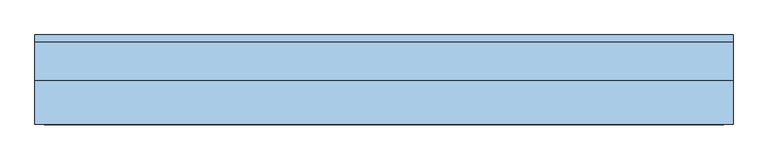
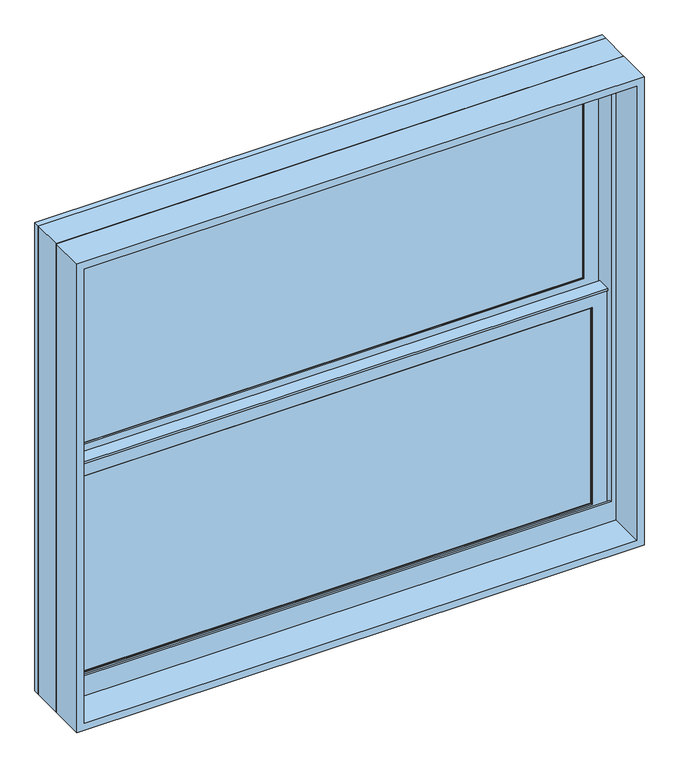
"""IFC4 building model written with IfcOpenShell, lengths in millimetres: window geometry, Window-Double_Hung-Marvin-Essential : ESDH4036."""

import ifcopenshell
import ifcopenshell.guid

model = None  # the IFC model being written
_history = None  # IfcOwnerHistory: only IFC2X3 demands one
_inside = {}  # id of a spatial element -> (the spatial element, [elements in it])
_under = {}  # id of a project, library or spatial element -> (it, [spatial elements below it])
_declared = {}  # id of a project -> (the project, [libraries it declares])
_typed = {}  # id of a type object -> (the type object, [elements of that type])
_made_of = {}  # id of a material, layer set ... -> (it, [elements and type objects made of it])


def new_model(schema):
    """Start an empty IFC model of exactly this schema.

    Asked for "IFC4X3", IfcOpenShell would pick the latest addendum, in which some entities
    have other attributes; the version numbers below select the first issue.
    IFC2X3 requires an IfcOwnerHistory on every rooted entity: one is made here for all.
    """
    global model, _history
    if schema == "IFC4X3":
        model = ifcopenshell.file(schema_version=(4, 3, 0, 0))
    else:
        model = ifcopenshell.file(schema=schema)
    _inside.clear()
    _under.clear()
    _declared.clear()
    _typed.clear()
    _made_of.clear()
    _history = None
    if model.schema == "IFC2X3":
        org = make("IfcOrganization", Name="unknown")
        user = make(
            "IfcPersonAndOrganization",
            ThePerson=make("IfcPerson", FamilyName="unknown"),
            TheOrganization=org,
        )
        app = make(
            "IfcApplication",
            ApplicationDeveloper=org,
            Version="unknown",
            ApplicationFullName="unknown",
            ApplicationIdentifier="unknown",
        )
        _history = make(
            "IfcOwnerHistory",
            OwningUser=user,
            OwningApplication=app,
            ChangeAction="ADDED",
            CreationDate=0,
        )
    return model


def make(cls, **values):
    """One entity of the class cls with the attributes given. An attribute that is None is left unset."""
    return model.create_entity(
        cls, **{name: value for name, value in values.items() if value is not None}
    )


def rooted(cls, **values):
    """An entity with a GlobalId (a new one), such as an element, a storey or a relation."""
    return make(cls, GlobalId=ifcopenshell.guid.new(), OwnerHistory=_history, **values)


def si_unit(unit_type, name, prefix=None):
    """IfcSIUnit, for example si_unit("LENGTHUNIT", "METRE", prefix="MILLI")."""
    return make("IfcSIUnit", UnitType=unit_type, Prefix=prefix, Name=name)


def assignment(units):
    """IfcUnitAssignment: the units of a project."""
    return None if units is None else make("IfcUnitAssignment", Units=units)


def point(xyz):
    """IfcCartesianPoint."""
    return None if xyz is None else make("IfcCartesianPoint", Coordinates=xyz)


def direction(xyz):
    """IfcDirection."""
    return None if xyz is None else make("IfcDirection", DirectionRatios=xyz)


def frame(location, z_axis=None, x_axis=None):
    """IfcAxis2Placement3D, a coordinate frame: its origin and axes. An axis left out is left unset."""
    return make(
        "IfcAxis2Placement3D",
        Location=point(location),
        Axis=direction(z_axis),
        RefDirection=direction(x_axis),
    )


def origin():
    """The frame at (0, 0, 0) with its axes left unset."""
    return frame((0.0, 0.0, 0.0))


def place(relative_to, where):
    """IfcLocalPlacement: puts the frame where relative to a parent placement (None: the world)."""
    return make(
        "IfcLocalPlacement", PlacementRelTo=relative_to, RelativePlacement=where
    )


def context(
    kind, dimensions, precision=None, world=None, true_north=None, identifier=None
):
    """IfcGeometricRepresentationContext, for example the 3D "Model" context."""
    return make(
        "IfcGeometricRepresentationContext",
        ContextIdentifier=identifier,
        ContextType=kind,
        CoordinateSpaceDimension=dimensions,
        Precision=precision,
        WorldCoordinateSystem=world,
        TrueNorth=true_north,
    )


def project(units=None, contexts=None):
    """IfcProject with its units and contexts."""
    return rooted(
        "IfcProject",
        Name="project",
        RepresentationContexts=contexts,
        UnitsInContext=assignment(units),
    )


def spatial(cls, under=None, at=None, **own):
    """A site, building, storey or space (cls), placed at a placement, below another one or the project."""
    s = rooted(cls, ObjectPlacement=at, **own)
    if under is not None:
        _under.setdefault(under.id(), (under, []))[1].append(s)
    return s


def polyline(points):
    """IfcPolyline through the points."""
    return make("IfcPolyline", Points=[point(p) for p in points])


def outline(outer, holes=None, kind="AREA"):
    """IfcArbitraryClosedProfileDef: a profile drawn as a closed curve; with holes, ...WithVoids."""
    if holes is None:
        return make("IfcArbitraryClosedProfileDef", ProfileType=kind, OuterCurve=outer)
    return make(
        "IfcArbitraryProfileDefWithVoids",
        ProfileType=kind,
        OuterCurve=outer,
        InnerCurves=holes,
    )


def extrude(swept, where, along, depth):
    """IfcExtrudedAreaSolid: the profile swept, set in the frame where, extruded along a direction by depth."""
    return make(
        "IfcExtrudedAreaSolid",
        SweptArea=swept,
        Position=where,
        ExtrudedDirection=direction(along),
        Depth=depth,
    )


def faces_of(points, faces, orient=None, outer=None):
    """IfcFace entities. A face is a list of loops; a loop is a list of indices into points, from 0.

    orient and outer hold one flag for each loop. By default every Orientation is true, the
    first loop of a face is its IfcFaceOuterBound and the others are IfcFaceBound.
    """
    made = []
    for i, loops in enumerate(faces):
        bounds = []
        for j, loop in enumerate(loops):
            is_outer = j == 0 if outer is None else outer[i][j]
            bounds.append(
                make(
                    "IfcFaceOuterBound" if is_outer else "IfcFaceBound",
                    Bound=make("IfcPolyLoop", Polygon=[points[k] for k in loop]),
                    Orientation=True if orient is None else orient[i][j],
                )
            )
        made.append(make("IfcFace", Bounds=bounds))
    return made


def faceted_brep(points, faces, orient=None, outer=None, voids=None):
    """IfcFacetedBrep: a solid bounded by flat faces; with voids (closed shells), ...WithVoids."""
    shared = [point(p) for p in points]
    hull = make("IfcClosedShell", CfsFaces=faces_of(shared, faces, orient, outer))
    if voids is None:
        return make("IfcFacetedBrep", Outer=hull)
    return make(
        "IfcFacetedBrepWithVoids",
        Outer=hull,
        Voids=[
            make(cls, CfsFaces=faces_of(shared, fs, o, b)) for cls, fs, o, b in voids
        ],
    )


def shape(context_of_items, identifier, shape_type, items):
    """IfcShapeRepresentation: the items that make up one representation, for example the "Body"."""
    return make(
        "IfcShapeRepresentation",
        ContextOfItems=context_of_items,
        RepresentationIdentifier=identifier,
        RepresentationType=shape_type,
        Items=items,
    )


def source(mapping_origin, context_of_items, identifier, shape_type, items):
    """IfcRepresentationMap: a shape defined once, which mapped items show again and again."""
    return make(
        "IfcRepresentationMap",
        MappingOrigin=mapping_origin,
        MappedRepresentation=shape(context_of_items, identifier, shape_type, items),
    )


def transform(
    local_origin,
    x_axis=None,
    y_axis=None,
    z_axis=None,
    scale=None,
    scale2=None,
    scale3=None,
    uniform=True,
):
    """IfcCartesianTransformationOperator3D, or its non-uniform kind. x_axis, y_axis, z_axis: its Axis1, 2, 3."""
    if uniform:
        return make(
            "IfcCartesianTransformationOperator3D",
            Axis1=direction(x_axis),
            Axis2=direction(y_axis),
            LocalOrigin=point(local_origin),
            Scale=scale,
            Axis3=direction(z_axis),
        )
    return make(
        "IfcCartesianTransformationOperator3DnonUniform",
        Axis1=direction(x_axis),
        Axis2=direction(y_axis),
        LocalOrigin=point(local_origin),
        Scale=scale,
        Axis3=direction(z_axis),
        Scale2=scale2,
        Scale3=scale3,
    )


def mapped(mapping_source, mapping_target):
    """IfcMappedItem: shows the shape of a source again, moved by a transform."""
    return make(
        "IfcMappedItem", MappingSource=mapping_source, MappingTarget=mapping_target
    )


def made_of(thing, what):
    """Note that an element or type object is made of a material, layer set ...; save() writes the relation."""
    if what is not None:
        _made_of.setdefault(what.id(), (what, []))[1].append(thing)
    return thing


def element(
    cls,
    number,
    at=None,
    inside=None,
    cuts=None,
    type_object=None,
    material=None,
    context=None,
    identifier="Body",
    shape_type=None,
    held_by="IfcProductDefinitionShape",
    body=None,
    shapes=None,
    **own,
):
    """One element of the class cls, such as IfcWall. Its Tag is "e" and its number.

    at: its placement. inside: the storey or other place that contains it. cuts: it is an
    opening in that element (IfcRelVoidsElement). A single representation is given by context,
    identifier, shape_type and body (its items); several are given by shapes. held_by: the class
    of the entity that holds the representations. save() writes the other relations.
    """
    e = rooted(cls, Tag="e%d" % number, ObjectPlacement=at, **own)
    if body is not None:
        shapes = [shape(context, identifier, shape_type, body)]
    if shapes is not None:
        e.Representation = make(held_by, Representations=shapes)
    if inside is not None:
        _inside.setdefault(inside.id(), (inside, []))[1].append(e)
    if cuts is not None:
        rooted(
            "IfcRelVoidsElement", RelatingBuildingElement=cuts, RelatedOpeningElement=e
        )
    if type_object is not None:
        _typed.setdefault(type_object.id(), (type_object, []))[1].append(e)
    return made_of(e, material)


def aggregate(whole, parts):
    """IfcRelAggregates: a whole, such as a stair, and the parts it consists of."""
    return rooted("IfcRelAggregates", RelatingObject=whole, RelatedObjects=parts)


def save(model, path):
    """Write the relations noted so far, then the file.

    IfcRelAggregates (storeys below a building ...), IfcRelContainedInSpatialStructure (elements
    in a storey), IfcRelDefinesByType, IfcRelAssociatesMaterial and IfcRelDeclares: one each for
    every whole, place, type object, material and project.
    """
    for whole, parts in _under.values():
        aggregate(whole, parts)
    for where, things in _inside.values():
        rooted(
            "IfcRelContainedInSpatialStructure",
            RelatedElements=things,
            RelatingStructure=where,
        )
    for kind, things in _typed.values():
        rooted("IfcRelDefinesByType", RelatedObjects=things, RelatingType=kind)
    for what, things in _made_of.values():
        rooted("IfcRelAssociatesMaterial", RelatedObjects=things, RelatingMaterial=what)
    for by, libraries in _declared.values():
        rooted("IfcRelDeclares", RelatingContext=by, RelatedDefinitions=libraries)
    model.write(path)


def window_972043b9(model_context):
    return source(origin(), model_context, "Body", "SolidModel", [
        extrude(outline(polyline([(191.5583333, 20.6375), (191.5583333, 15.875), (172.5083333, 15.875), (172.5083333, 20.6375), (191.5583333, 20.6375)])), frame((0.0, 0.0, 1441.45), z_axis=(0.0, 0.0, 1.0), x_axis=(1.0, 0.0, 0.0)), (0.0, 0.0, 1.0), 450.85),
        extrude(outline(polyline([(-172.5083333, 20.6375), (-172.5083333, 15.875), (-191.5583333, 15.875), (-191.5583333, 20.6375), (-172.5083333, 20.6375)])), frame((0.0, 0.0, 1441.45), z_axis=(0.0, 0.0, 1.0), x_axis=(1.0, 0.0, 0.0)), (0.0, 0.0, 1.0), 450.85),
        extrude(outline(polyline([(546.1, 20.6375), (546.1, 15.875), (-546.1, 15.875), (-546.1, 20.6375), (546.1, 20.6375)])), frame((0.0, 0.0, 1657.35), z_axis=(0.0, 0.0, 1.0), x_axis=(1.0, 0.0, 0.0)), (0.0, 0.0, 1.0), 19.05),
        extrude(outline(polyline([(-191.5583333, 46.83125), (-191.5583333, 51.59375), (-172.5083333, 51.59375), (-172.5083333, 46.83125), (-191.5583333, 46.83125)])), frame((0.0, 0.0, 1930.4), z_axis=(0.0, 0.0, 1.0), x_axis=(1.0, 0.0, 0.0)), (0.0, 0.0, 1.0), 450.85),
        extrude(outline(polyline([(172.5083333, 46.83125), (172.5083333, 51.59375), (191.5583333, 51.59375), (191.5583333, 46.83125), (172.5083333, 46.83125)])), frame((0.0, 0.0, 1930.4), z_axis=(0.0, 0.0, 1.0), x_axis=(1.0, 0.0, 0.0)), (0.0, 0.0, 1.0), 450.85),
        extrude(outline(polyline([(-546.1, 46.83125), (-546.1, 51.59375), (546.1, 51.59375), (546.1, 46.83125), (-546.1, 46.83125)])), frame((0.0, 0.0, 2146.3), z_axis=(0.0, 0.0, 1.0), x_axis=(1.0, 0.0, 0.0)), (0.0, 0.0, 1.0), 19.05),
        extrude(outline(polyline([(191.5583333, 20.6375), (172.5083333, 20.6375), (172.5083333, 25.4), (191.5583333, 25.4), (191.5583333, 20.6375)])), frame((0.0, 0.0, 1441.45), z_axis=(0.0, 0.0, 1.0), x_axis=(1.0, 0.0, 0.0)), (0.0, 0.0, 1.0), 450.85),
        extrude(outline(polyline([(-172.5083333, 20.6375), (-191.5583333, 20.6375), (-191.5583333, 25.4), (-172.5083333, 25.4), (-172.5083333, 20.6375)])), frame((0.0, 0.0, 1441.45), z_axis=(0.0, 0.0, 1.0), x_axis=(1.0, 0.0, 0.0)), (0.0, 0.0, 1.0), 450.85),
        extrude(outline(polyline([(546.1, 20.6375), (-546.1, 20.6375), (-546.1, 25.4), (546.1, 25.4), (546.1, 20.6375)])), frame((0.0, 0.0, 1657.35), z_axis=(0.0, 0.0, 1.0), x_axis=(1.0, 0.0, 0.0)), (0.0, 0.0, 1.0), 19.05),
        extrude(outline(polyline([(-191.5583333, 56.35625), (-172.5083333, 56.35625), (-172.5083333, 51.59375), (-191.5583333, 51.59375), (-191.5583333, 56.35625)])), frame((0.0, 0.0, 1930.4), z_axis=(0.0, 0.0, 1.0), x_axis=(1.0, 0.0, 0.0)), (0.0, 0.0, 1.0), 450.85),
        extrude(outline(polyline([(172.5083333, 56.35625), (191.5583333, 56.35625), (191.5583333, 51.59375), (172.5083333, 51.59375), (172.5083333, 56.35625)])), frame((0.0, 0.0, 1930.4), z_axis=(0.0, 0.0, 1.0), x_axis=(1.0, 0.0, 0.0)), (0.0, 0.0, 1.0), 450.85),
        extrude(outline(polyline([(-546.1, 56.35625), (546.1, 56.35625), (546.1, 51.59375), (-546.1, 51.59375), (-546.1, 56.35625)])), frame((0.0, 0.0, 2146.3), z_axis=(0.0, 0.0, 1.0), x_axis=(1.0, 0.0, 0.0)), (0.0, 0.0, 1.0), 19.05),
        faceted_brep([(-573.0875, 5.6780605, 1922.3351748), (-573.0875, 5.6780605, 1917.7), (573.0875, 5.6780605, 1917.7), (573.0875, 5.6780605, 1922.3351748), (-573.0875, 34.8118605, 1922.3351748), (573.0875, 34.8118605, 1922.3351748), (573.0875, 34.8118605, 1917.7), (-573.0875, 34.8118605, 1917.7), (-573.0875, 30.1625, 1917.7), (-573.0875, 30.1625, 1414.4625), (-573.0875, 8.9241104, 1414.4625), (-573.0875, 8.9241104, 1917.7), (573.0875, 8.9241104, 1917.7), (573.0875, 30.1625, 1917.7), (573.0875, 8.9241104, 1414.4625), (573.0875, 30.1625, 1414.4625), (-557.2034752, 11.90625, 1903.4034752), (-557.2034752, 30.1625, 1903.4034752), (557.2034752, 30.1625, 1903.4034752), (557.2034752, 11.90625, 1903.4034752), (-540.54375, 10.4662439, 1886.74375), (-540.54375, 11.90625, 1886.74375), (540.54375, 11.90625, 1886.74375), (540.54375, 10.4662439, 1886.74375), (542.0858834, 8.9241104, 1888.2858834), (-542.0858834, 8.9241104, 1888.2858834), (557.2034752, 30.1625, 1430.3465248), (557.2034752, 11.90625, 1430.3465248), (540.54375, 11.90625, 1447.00625), (540.54375, 10.4662439, 1447.00625), (542.0858834, 8.9241104, 1445.4641166), (-557.2034752, 30.1625, 1430.3465248), (-557.2034752, 11.90625, 1430.3465248), (-540.54375, 11.90625, 1447.00625), (-540.54375, 10.4662439, 1447.00625), (-542.0858834, 8.9241104, 1445.4641166)], [[[0, 1, 2, 3]], [[4, 5, 6, 7]], [[1, 0, 4, 7, 8, 9, 10, 11]], [[2, 1, 11, 12]], [[7, 6, 13, 8]], [[3, 2, 12, 14, 15, 13, 6, 5]], [[0, 3, 5, 4]], [[16, 17, 18, 19]], [[20, 21, 22, 23]], [[20, 23, 24, 25]], [[19, 18, 26, 27]], [[23, 22, 28, 29]], [[24, 23, 29, 30]], [[27, 26, 31, 32]], [[29, 28, 33, 34]], [[30, 29, 34, 35]], [[15, 14, 10, 9]], [[15, 9, 8, 13], [18, 17, 31, 26]], [[17, 16, 32, 31]], [[16, 19, 27, 32], [22, 21, 33, 28]], [[21, 20, 34, 33]], [[20, 25, 35, 34]], [[10, 14, 12, 11], [25, 24, 30, 35]]]),
        extrude(outline(polyline([(38.5955581, 1903.4125), (33.5778968, 1903.4125), (33.5778968, 1905.0), (39.9405976, 1905.0), (39.9405976, 1903.4125), (61.515625, 1903.4125), (47.6307501, 1900.0975159), (38.5955581, 1900.0975159), (38.5955581, 1903.4125)])), frame((-573.0875, 0.0, 0.0), z_axis=(1.0, 0.0, 0.0), x_axis=(0.0, 1.0, 0.0)), (0.0, 0.0, 1.0), 1146.175),
        faceted_brep([(603.25, 0.0, 1384.3), (603.25, 0.0, 2438.4), (-603.25, 0.0, 2438.4), (-603.25, 0.0, 1384.3), (577.05625, 0.0, 1445.41875), (-577.05625, 0.0, 1445.41875), (-577.05625, 0.0, 2412.20625), (577.05625, 0.0, 2412.20625), (577.05625, 3.96875, 1384.3), (-577.05625, 3.96875, 1384.3), (-577.05625, 3.96875, 1445.41875), (577.05625, 3.96875, 1445.41875), (-603.25, 65.6828125, 1384.3), (-577.05625, 65.6828125, 1384.3), (577.05625, 65.6828125, 1384.3), (603.25, 65.6828125, 1384.3), (-603.25, 65.6828125, 2438.4), (603.25, 65.6828125, 2438.4), (577.05625, 65.6828125, 2412.20625), (-577.05625, 65.6828125, 2412.20625)], [[[0, 1, 2, 3], [4, 5, 6, 7]], [[8, 9, 10, 11]], [[5, 4, 11, 10]], [[0, 3, 12, 13, 9, 8, 14, 15]], [[13, 12, 16, 17, 15, 14, 18, 19]], [[13, 19, 6, 5, 10, 9]], [[7, 6, 19, 18]], [[18, 14, 8, 11, 4, 7]], [[1, 0, 15, 17]], [[2, 1, 17, 16]], [[3, 2, 16, 12]]]),
        faceted_brep([(577.05625, 30.1625, 1911.35), (575.46875, 30.1625, 1911.35), (575.46875, 30.1625, 1408.6544613), (577.05625, 30.1625, 1408.6544613), (-575.46875, 30.1625, 1911.35), (-577.05625, 30.1625, 1911.35), (-577.05625, 30.1625, 1408.6544613), (-575.46875, 30.1625, 1408.6544613), (575.46875, 63.5, 1911.35), (577.05625, 63.5, 1911.35), (577.05625, 63.5, 1402.1743077), (575.46875, 63.5, 1402.1743077), (-577.05625, 63.5, 1911.35), (-575.46875, 63.5, 1911.35), (-575.46875, 63.5, 1402.1743077), (-577.05625, 63.5, 1402.1743077), (588.3108932, 3.96875, 1413.7460105), (588.3108932, 3.96875, 1384.3), (588.3108932, 65.6828125, 1384.3), (588.3108932, 65.6828125, 1401.750012), (-588.3108932, 3.96875, 1384.3), (-588.3108932, 3.96875, 1413.7460105), (-588.3108932, 65.6828125, 1401.750012), (-588.3108932, 65.6828125, 1384.3), (588.3108932, 78.58125, 1399.2428097), (-588.3108932, 78.58125, 1399.2428097), (-586.2971252, 68.2348864, 1401.2539391), (-568.33135, 68.2348864, 1401.2539391), (-568.33135, 65.6828125, 1401.750012), (568.33135, 65.6828125, 1401.750012), (568.33135, 68.2348864, 1401.2539391), (586.2971252, 68.2348864, 1401.2539391), (-603.25, 65.6828125, 1384.3), (-603.25, 78.5948249, 1384.3), (603.25, 78.5948249, 1384.3), (603.25, 65.6828125, 1384.3), (-603.25, 78.58125, 2438.4), (603.25, 78.58125, 2438.4), (588.3108932, 78.58125, 2423.4608932), (-588.3108932, 78.58125, 2423.4608932), (-603.25, 65.6828125, 2438.4), (-586.2971252, 68.2348864, 2421.4471252), (586.2971252, 68.2348864, 2421.4471252), (568.33135, 68.2348864, 2403.48135), (-568.33135, 68.2348864, 2403.48135), (-568.33135, 65.6828125, 2403.48135), (568.33135, 65.6828125, 2403.48135), (603.25, 65.6828125, 2438.4)], [[[0, 1, 2, 3]], [[4, 5, 6, 7]], [[8, 9, 10, 11]], [[12, 13, 14, 15]], [[1, 8, 11, 2]], [[9, 0, 3, 10]], [[1, 0, 9, 8]], [[5, 4, 13, 12]], [[5, 12, 15, 6]], [[13, 4, 7, 14]], [[16, 17, 18, 19]], [[20, 21, 22, 23]], [[24, 25, 26, 27, 28, 22, 21, 16, 19, 29, 30, 31], [3, 2, 11, 10], [7, 6, 15, 14]], [[17, 16, 21, 20]], [[17, 20, 23, 32, 33, 34, 35, 18]], [[34, 33, 36, 37], [25, 24, 38, 39]], [[33, 32, 40, 36]], [[39, 41, 26, 25]], [[41, 42, 31, 30, 43, 44, 27, 26]], [[44, 45, 28, 27]], [[40, 32, 23, 22, 28, 45, 46, 29, 19, 18, 35, 47]], [[36, 40, 47, 37]], [[39, 38, 42, 41]], [[44, 43, 46, 45]], [[34, 37, 47, 35]], [[42, 38, 24, 31]], [[46, 43, 30, 29]]]),
        extrude(outline(polyline([(553.24375, 11.90625), (-553.24375, 11.90625), (-553.24375, 15.08125), (553.24375, 15.08125), (553.24375, 11.90625)])), frame((0.0, 0.0, 1434.30625), z_axis=(0.0, 0.0, 1.0), x_axis=(1.0, 0.0, 0.0)), (0.0, 0.0, 1.0), 465.1375),
        extrude(outline(polyline([(553.24375, 42.8625), (-553.24375, 42.8625), (-553.24375, 46.0375), (553.24375, 46.0375), (553.24375, 42.8625)])), frame((0.0, 0.0, 1923.25625), z_axis=(0.0, 0.0, 1.0), x_axis=(1.0, 0.0, 0.0)), (0.0, 0.0, 1.0), 465.1375),
        faceted_brep([(-540.54375, 31.194477, 1886.74375), (-542.0858834, 32.7366104, 1888.2858834), (542.0858834, 32.7366104, 1888.2858834), (540.54375, 31.194477, 1886.74375), (-540.54375, 30.1625, 1886.74375), (540.54375, 30.1625, 1886.74375), (-573.0875, 32.7366104, 1919.2875), (-573.0875, 30.1625, 1919.2875), (573.0875, 30.1625, 1919.2875), (573.0875, 32.7366104, 1919.2875), (542.0858834, 32.7366104, 1445.4641166), (540.54375, 31.194477, 1447.00625), (540.54375, 30.1625, 1447.00625), (573.0875, 30.1625, 1414.4625), (573.0875, 32.7366104, 1414.4625), (-542.0858834, 32.7366104, 1445.4641166), (-540.54375, 31.194477, 1447.00625), (-540.54375, 30.1625, 1447.00625), (-573.0875, 30.1625, 1414.4625), (-573.0875, 32.7366104, 1414.4625)], [[[0, 1, 2, 3]], [[4, 0, 3, 5]], [[6, 7, 8, 9]], [[3, 2, 10, 11]], [[5, 3, 11, 12]], [[9, 8, 13, 14]], [[11, 10, 15, 16]], [[12, 11, 16, 17]], [[14, 13, 18, 19]], [[9, 14, 19, 6], [1, 15, 10, 2]], [[16, 15, 1, 0]], [[17, 16, 0, 4]], [[7, 18, 13, 8], [5, 12, 17, 4]], [[19, 18, 7, 6]]]),
        faceted_brep([(-557.2034752, 42.8625, 2392.3534752), (-557.2034752, 61.11875, 2392.3534752), (557.2034752, 61.11875, 2392.3534752), (557.2034752, 42.8625, 2392.3534752), (-540.54375, 41.4224939, 2375.69375), (-540.54375, 42.8625, 2375.69375), (540.54375, 42.8625, 2375.69375), (540.54375, 41.4224939, 2375.69375), (-542.0858834, 39.8803604, 2377.2358834), (542.0858834, 39.8803604, 2377.2358834), (-573.0875, 61.11875, 2408.2375), (-573.0875, 39.8803604, 2408.2375), (573.0875, 39.8803604, 2408.2375), (573.0875, 61.11875, 2408.2375), (557.2034752, 61.11875, 1919.2965248), (557.2034752, 42.8625, 1919.2965248), (540.54375, 42.8625, 1935.95625), (540.54375, 41.4224939, 1935.95625), (542.0858834, 39.8803604, 1934.4141166), (573.0875, 39.8803604, 1903.4125), (573.0875, 61.11875, 1903.4125), (-557.2034752, 61.11875, 1919.2965248), (-557.2034752, 42.8625, 1919.2965248), (-540.54375, 42.8625, 1935.95625), (-540.54375, 41.4224939, 1935.95625), (-542.0858834, 39.8803604, 1934.4141166), (-573.0875, 39.8803604, 1903.4125), (-573.0875, 61.11875, 1903.4125)], [[[0, 1, 2, 3]], [[4, 5, 6, 7]], [[8, 4, 7, 9]], [[10, 11, 12, 13]], [[3, 2, 14, 15]], [[7, 6, 16, 17]], [[9, 7, 17, 18]], [[13, 12, 19, 20]], [[15, 14, 21, 22]], [[17, 16, 23, 24]], [[18, 17, 24, 25]], [[20, 19, 26, 27]], [[13, 20, 27, 10], [1, 21, 14, 2]], [[22, 21, 1, 0]], [[3, 15, 22, 0], [5, 23, 16, 6]], [[24, 23, 5, 4]], [[25, 24, 4, 8]], [[11, 26, 19, 12], [9, 18, 25, 8]], [[27, 26, 11, 10]]]),
        faceted_brep([(-573.0875, 61.11875, 1903.4125), (-573.0875, 63.6928604, 1903.4125), (573.0875, 63.6928604, 1903.4125), (573.0875, 61.11875, 1903.4125), (-540.54375, 62.150727, 1935.95625), (-540.54375, 61.11875, 1935.95625), (540.54375, 61.11875, 1935.95625), (540.54375, 62.150727, 1935.95625), (-542.0858834, 63.6928604, 1934.4141166), (542.0858834, 63.6928604, 1934.4141166), (573.0875, 63.6928604, 2408.2375), (573.0875, 61.11875, 2408.2375), (540.54375, 61.11875, 2375.69375), (540.54375, 62.150727, 2375.69375), (542.0858834, 63.6928604, 2377.2358834), (-573.0875, 63.6928604, 2408.2375), (-573.0875, 61.11875, 2408.2375), (-540.54375, 61.11875, 2375.69375), (-540.54375, 62.150727, 2375.69375), (-542.0858834, 63.6928604, 2377.2358834)], [[[0, 1, 2, 3]], [[4, 5, 6, 7]], [[8, 4, 7, 9]], [[3, 2, 10, 11]], [[7, 6, 12, 13]], [[9, 7, 13, 14]], [[11, 10, 15, 16]], [[13, 12, 17, 18]], [[14, 13, 18, 19]], [[16, 15, 1, 0]], [[3, 11, 16, 0], [5, 17, 12, 6]], [[18, 17, 5, 4]], [[19, 18, 4, 8]], [[1, 15, 10, 2], [9, 14, 19, 8]]]),
        extrude(outline(polyline([(553.24375, 26.19375), (-553.24375, 26.19375), (-553.24375, 30.1625), (553.24375, 30.1625), (553.24375, 26.19375)])), frame((0.0, 0.0, 1434.30625), z_axis=(0.0, 0.0, 1.0), x_axis=(1.0, 0.0, 0.0)), (0.0, 0.0, 1.0), 465.1375),
        extrude(outline(polyline([(553.24375, 57.15), (-553.24375, 57.15), (-553.24375, 61.11875), (553.24375, 61.11875), (553.24375, 57.15)])), frame((0.0, 0.0, 1923.25625), z_axis=(0.0, 0.0, 1.0), x_axis=(1.0, 0.0, 0.0)), (0.0, 0.0, 1.0), 465.1375),
        extrude(outline(polyline([(2438.4, 603.25), (2438.4, -603.25), (1384.3, -603.25), (1384.3, 603.25), (2438.4, 603.25)]), holes=[polyline([(2422.525, 587.375), (1400.175, 587.375), (1400.175, -587.375), (2422.525, -587.375), (2422.525, 587.375)])]), frame((0.0, -76.2, 0.0), z_axis=(0.0, 1.0, 0.0), x_axis=(0.0, 0.0, 1.0)), (0.0, 0.0, 1.0), 75.40625),
    ])


if __name__ == "__main__":
    model = new_model("IFC4")
    model_context = context("Model", 3, world=origin())
    ifc_project = project(units=[si_unit("LENGTHUNIT", "METRE", prefix="MILLI")], contexts=[model_context])
    site = spatial("IfcSite", under=ifc_project)
    building = spatial("IfcBuilding", under=site)
    placement = place(None, origin())
    window_shape = window_972043b9(model_context)
    element("IfcWindow", 1, ObjectType="Window-Double_Hung-Marvin-Essential : ESDH4036", at=placement, inside=building, context=model_context, shape_type="MappedRepresentation", body=[
        mapped(window_shape, transform((0.0, 0.0, 0.0), x_axis=(1.0, 0.0, 0.0), y_axis=(0.0, 1.0, 0.0), z_axis=(0.0, 0.0, 1.0))),
    ])
    save(model, "model.ifc")

# Revit data of these elements
# Type "Window-Double_Hung-Marvin-Essential : ESDH4036"
#   Type Mark = "46"
#   Window Type = "Essential Double Hung"
#   Product data url = "https://bimobject.com/marvin-windows-and-doors/product/marvin-dhwau"
#   Product Guid = "c4a96547-874c-4385-91dc-a058adc19d98"
#   Frame = "All Ultrex"
#   Egress Window = "No"
#   URL = "www.marvin.com"
#   Model = "ESDH4036"
#   Manufacturer = "Marvin Windows and Doors"
#   Label Egress = ""
#   Glass Type = "IG Low E II with Argon"
#   Design Pressure = "DP50"
#   Description = "4842 DBHG"
#   Analytic Construction = "<None>"
#   Prairie Corner Width = 0' - 4"
#   Prairie Corner Height = 0' - 4"
#   Egress Width = 3' - 8 9/16"
#   Egress Height = 1' - 4 27/128"
#   Rough Width = 4' - 0"
#   Rough Height = 3' - 6"
#   Nominal Width = 4' - 0"
#   Nominal Height = 3' - 6"
#   Inset to Installation Flange [instance default] = 0' - 1"
#   Height = 3' - 5 1/2"
#   Egress Area = 5.01667 SF
#   Default Head Height = 8' - 0"
#   Width = 3' - 11 1/2"
#   Daylight Area = 10.2342 SF
#   DLO Width = 3' - 6 9/16"
#   DLO Height = 1' - 5 5/16"
#   Muntins Top Sash = yes
#   Lites Wide Top Sash = 3
#   Lites Wide Bottom Sash = 3
#   Lites High Top Sash = 2
#   Lites High Bottom Sash = 2
#   Lite Cut Prairie 9 = no
#   Lite Cut HV Grid = yes
#   Muntins Bottom Sash = yes
#   Label Visibility = no
#   Jamb Extension Visibility = yes
#   Edition number = 1
#   Interior Material = Ultrex-Marvin-Stonewhite
#   Glazing Material = Glass-Marvin-IG Low E II with Argon
#   Cladding Material = Ultrex-Marvin-Pebblegray
#   Wall Closure = (empty or 0)
#   Assembly Code = ""
# Element 1 (IfcWindow, "Window-Double_Hung-Marvin-Essential : ESDH4036")
#   Materials on its faces: "Ultrex-Marvin-Pebblegray", "Ultrex-Marvin-Stonewhite", "Glass-Marvin-IG Low E II with Argon"
# Materials
#   "Ultrex-Marvin-Stonewhite": class "Paint", colour RGB 250 251 245, transparency 0
#   "Glass-Marvin-IG Low E II with Argon": class "Glass", colour RGB 0 128 192, transparency 0.85
#   "Ultrex-Marvin-Pebblegray": class "Paint", colour RGB 189 185 173, transparency 0
